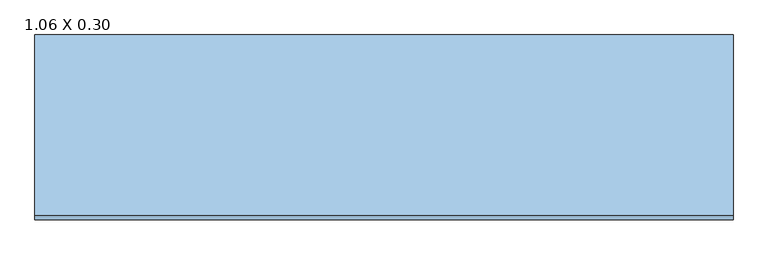
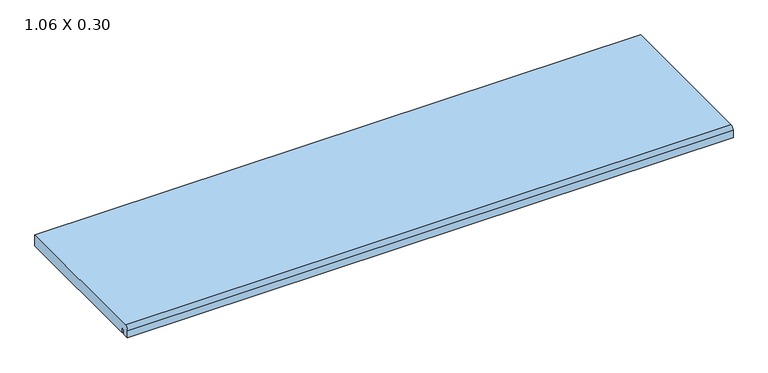
"""IFC4 building model written with IfcOpenShell, lengths in millimetres: window geometry, .CC_ND 300_PEDRA_PEITORIL RETO : 1.06 X 0.30."""

import ifcopenshell
import ifcopenshell.guid

model = None  # the IFC model being written
_history = None  # IfcOwnerHistory: only IFC2X3 demands one
_inside = {}  # id of a spatial element -> (the spatial element, [elements in it])
_under = {}  # id of a project, library or spatial element -> (it, [spatial elements below it])
_declared = {}  # id of a project -> (the project, [libraries it declares])
_typed = {}  # id of a type object -> (the type object, [elements of that type])
_made_of = {}  # id of a material, layer set ... -> (it, [elements and type objects made of it])


def new_model(schema):
    """Start an empty IFC model of exactly this schema.

    Asked for "IFC4X3", IfcOpenShell would pick the latest addendum, in which some entities
    have other attributes; the version numbers below select the first issue.
    IFC2X3 requires an IfcOwnerHistory on every rooted entity: one is made here for all.
    """
    global model, _history
    if schema == "IFC4X3":
        model = ifcopenshell.file(schema_version=(4, 3, 0, 0))
    else:
        model = ifcopenshell.file(schema=schema)
    _inside.clear()
    _under.clear()
    _declared.clear()
    _typed.clear()
    _made_of.clear()
    _history = None
    if model.schema == "IFC2X3":
        org = make("IfcOrganization", Name="unknown")
        user = make(
            "IfcPersonAndOrganization",
            ThePerson=make("IfcPerson", FamilyName="unknown"),
            TheOrganization=org,
        )
        app = make(
            "IfcApplication",
            ApplicationDeveloper=org,
            Version="unknown",
            ApplicationFullName="unknown",
            ApplicationIdentifier="unknown",
        )
        _history = make(
            "IfcOwnerHistory",
            OwningUser=user,
            OwningApplication=app,
            ChangeAction="ADDED",
            CreationDate=0,
        )
    return model


def make(cls, **values):
    """One entity of the class cls with the attributes given. An attribute that is None is left unset."""
    return model.create_entity(
        cls, **{name: value for name, value in values.items() if value is not None}
    )


def rooted(cls, **values):
    """An entity with a GlobalId (a new one), such as an element, a storey or a relation."""
    return make(cls, GlobalId=ifcopenshell.guid.new(), OwnerHistory=_history, **values)


def si_unit(unit_type, name, prefix=None):
    """IfcSIUnit, for example si_unit("LENGTHUNIT", "METRE", prefix="MILLI")."""
    return make("IfcSIUnit", UnitType=unit_type, Prefix=prefix, Name=name)


def assignment(units):
    """IfcUnitAssignment: the units of a project."""
    return None if units is None else make("IfcUnitAssignment", Units=units)


def point(xyz):
    """IfcCartesianPoint."""
    return None if xyz is None else make("IfcCartesianPoint", Coordinates=xyz)


def direction(xyz):
    """IfcDirection."""
    return None if xyz is None else make("IfcDirection", DirectionRatios=xyz)


def frame(location, z_axis=None, x_axis=None):
    """IfcAxis2Placement3D, a coordinate frame: its origin and axes. An axis left out is left unset."""
    return make(
        "IfcAxis2Placement3D",
        Location=point(location),
        Axis=direction(z_axis),
        RefDirection=direction(x_axis),
    )


def frame_2d(location, x_axis=None):
    """IfcAxis2Placement2D, a coordinate frame in the plane: its origin and x axis."""
    return make(
        "IfcAxis2Placement2D", Location=point(location), RefDirection=direction(x_axis)
    )


def origin():
    """The frame at (0, 0, 0) with its axes left unset."""
    return frame((0.0, 0.0, 0.0))


def place(relative_to, where):
    """IfcLocalPlacement: puts the frame where relative to a parent placement (None: the world)."""
    return make(
        "IfcLocalPlacement", PlacementRelTo=relative_to, RelativePlacement=where
    )


def context(
    kind, dimensions, precision=None, world=None, true_north=None, identifier=None
):
    """IfcGeometricRepresentationContext, for example the 3D "Model" context."""
    return make(
        "IfcGeometricRepresentationContext",
        ContextIdentifier=identifier,
        ContextType=kind,
        CoordinateSpaceDimension=dimensions,
        Precision=precision,
        WorldCoordinateSystem=world,
        TrueNorth=true_north,
    )


def project(units=None, contexts=None):
    """IfcProject with its units and contexts."""
    return rooted(
        "IfcProject",
        Name="project",
        RepresentationContexts=contexts,
        UnitsInContext=assignment(units),
    )


def spatial(cls, under=None, at=None, **own):
    """A site, building, storey or space (cls), placed at a placement, below another one or the project."""
    s = rooted(cls, ObjectPlacement=at, **own)
    if under is not None:
        _under.setdefault(under.id(), (under, []))[1].append(s)
    return s


def polyline(points):
    """IfcPolyline through the points."""
    return make("IfcPolyline", Points=[point(p) for p in points])


def circle_curve(where, radius):
    """IfcCircle in the frame where."""
    return make("IfcCircle", Position=where, Radius=radius)


def trimmed(basis, trim1, trim2, sense, master):
    """IfcTrimmedCurve: the piece of a basis curve between two trims."""
    return make(
        "IfcTrimmedCurve",
        BasisCurve=basis,
        Trim1=trim1,
        Trim2=trim2,
        SenseAgreement=sense,
        MasterRepresentation=master,
    )


def segment(curve, same_sense, transition):
    """IfcCompositeCurveSegment."""
    return make(
        "IfcCompositeCurveSegment",
        Transition=transition,
        SameSense=same_sense,
        ParentCurve=curve,
    )


def composite_curve(segments, self_intersect=None):
    """IfcCompositeCurve: segments joined end to end."""
    return make("IfcCompositeCurve", Segments=segments, SelfIntersect=self_intersect)


def outline(outer, holes=None, kind="AREA"):
    """IfcArbitraryClosedProfileDef: a profile drawn as a closed curve; with holes, ...WithVoids."""
    if holes is None:
        return make("IfcArbitraryClosedProfileDef", ProfileType=kind, OuterCurve=outer)
    return make(
        "IfcArbitraryProfileDefWithVoids",
        ProfileType=kind,
        OuterCurve=outer,
        InnerCurves=holes,
    )


def extrude(swept, where, along, depth):
    """IfcExtrudedAreaSolid: the profile swept, set in the frame where, extruded along a direction by depth."""
    return make(
        "IfcExtrudedAreaSolid",
        SweptArea=swept,
        Position=where,
        ExtrudedDirection=direction(along),
        Depth=depth,
    )


def shape(context_of_items, identifier, shape_type, items):
    """IfcShapeRepresentation: the items that make up one representation, for example the "Body"."""
    return make(
        "IfcShapeRepresentation",
        ContextOfItems=context_of_items,
        RepresentationIdentifier=identifier,
        RepresentationType=shape_type,
        Items=items,
    )


def source(mapping_origin, context_of_items, identifier, shape_type, items):
    """IfcRepresentationMap: a shape defined once, which mapped items show again and again."""
    return make(
        "IfcRepresentationMap",
        MappingOrigin=mapping_origin,
        MappedRepresentation=shape(context_of_items, identifier, shape_type, items),
    )


def transform(
    local_origin,
    x_axis=None,
    y_axis=None,
    z_axis=None,
    scale=None,
    scale2=None,
    scale3=None,
    uniform=True,
):
    """IfcCartesianTransformationOperator3D, or its non-uniform kind. x_axis, y_axis, z_axis: its Axis1, 2, 3."""
    if uniform:
        return make(
            "IfcCartesianTransformationOperator3D",
            Axis1=direction(x_axis),
            Axis2=direction(y_axis),
            LocalOrigin=point(local_origin),
            Scale=scale,
            Axis3=direction(z_axis),
        )
    return make(
        "IfcCartesianTransformationOperator3DnonUniform",
        Axis1=direction(x_axis),
        Axis2=direction(y_axis),
        LocalOrigin=point(local_origin),
        Scale=scale,
        Axis3=direction(z_axis),
        Scale2=scale2,
        Scale3=scale3,
    )


def mapped(mapping_source, mapping_target):
    """IfcMappedItem: shows the shape of a source again, moved by a transform."""
    return make(
        "IfcMappedItem", MappingSource=mapping_source, MappingTarget=mapping_target
    )


def made_of(thing, what):
    """Note that an element or type object is made of a material, layer set ...; save() writes the relation."""
    if what is not None:
        _made_of.setdefault(what.id(), (what, []))[1].append(thing)
    return thing


def element(
    cls,
    number,
    at=None,
    inside=None,
    cuts=None,
    type_object=None,
    material=None,
    context=None,
    identifier="Body",
    shape_type=None,
    held_by="IfcProductDefinitionShape",
    body=None,
    shapes=None,
    **own,
):
    """One element of the class cls, such as IfcWall. Its Tag is "e" and its number.

    at: its placement. inside: the storey or other place that contains it. cuts: it is an
    opening in that element (IfcRelVoidsElement). A single representation is given by context,
    identifier, shape_type and body (its items); several are given by shapes. held_by: the class
    of the entity that holds the representations. save() writes the other relations.
    """
    e = rooted(cls, Tag="e%d" % number, ObjectPlacement=at, **own)
    if body is not None:
        shapes = [shape(context, identifier, shape_type, body)]
    if shapes is not None:
        e.Representation = make(held_by, Representations=shapes)
    if inside is not None:
        _inside.setdefault(inside.id(), (inside, []))[1].append(e)
    if cuts is not None:
        rooted(
            "IfcRelVoidsElement", RelatingBuildingElement=cuts, RelatedOpeningElement=e
        )
    if type_object is not None:
        _typed.setdefault(type_object.id(), (type_object, []))[1].append(e)
    return made_of(e, material)


def aggregate(whole, parts):
    """IfcRelAggregates: a whole, such as a stair, and the parts it consists of."""
    return rooted("IfcRelAggregates", RelatingObject=whole, RelatedObjects=parts)


def save(model, path):
    """Write the relations noted so far, then the file.

    IfcRelAggregates (storeys below a building ...), IfcRelContainedInSpatialStructure (elements
    in a storey), IfcRelDefinesByType, IfcRelAssociatesMaterial and IfcRelDeclares: one each for
    every whole, place, type object, material and project.
    """
    for whole, parts in _under.values():
        aggregate(whole, parts)
    for where, things in _inside.values():
        rooted(
            "IfcRelContainedInSpatialStructure",
            RelatedElements=things,
            RelatingStructure=where,
        )
    for kind, things in _typed.values():
        rooted("IfcRelDefinesByType", RelatedObjects=things, RelatingType=kind)
    for what, things in _made_of.values():
        rooted("IfcRelAssociatesMaterial", RelatedObjects=things, RelatingMaterial=what)
    for by, libraries in _declared.values():
        rooted("IfcRelDeclares", RelatingContext=by, RelatedDefinitions=libraries)
    model.write(path)


def window_1_06_x_0_30_ddfe798f(model_context):
    return source(origin(), model_context, "Body", "SweptSolid", [
        extrude(outline(composite_curve([segment(polyline([(-132.5083081, 1480.0), (-132.5083081, 1488.1993124), (-137.2619526, 1488.1993124), (-137.2619526, 1480.0), (-148.0, 1480.0), (-148.0, 1493.3808343)]), True, "CONTINUOUS"), segment(trimmed(circle_curve(frame_2d((-141.3808343, 1493.3808343)), 6.6191657), [point((-148.0, 1493.3808343))], [point((-141.3808343, 1500.0))], False, "CARTESIAN"), True, "CONTINUOUS"), segment(polyline([(-141.3808343, 1500.0), (132.7, 1500.0), (132.7, 1480.0), (-132.5083081, 1480.0)]), True, "CONTINUOUS")], self_intersect=False)), frame((-530.0, 0.0, 0.0), z_axis=(1.0, 0.0, 0.0), x_axis=(0.0, 1.0, 0.0)), (0.0, 0.0, 1.0), 1060.0),
    ])


if __name__ == "__main__":
    model = new_model("IFC4")
    model_context = context("Model", 3, world=origin())
    ifc_project = project(units=[si_unit("LENGTHUNIT", "METRE", prefix="MILLI")], contexts=[model_context])
    site = spatial("IfcSite", under=ifc_project)
    building = spatial("IfcBuilding", under=site)
    placement = place(None, origin())
    window_1_06_x_0_30_shape = window_1_06_x_0_30_ddfe798f(model_context)
    element("IfcWindow", 1, ObjectType=".CC_ND 300_PEDRA_PEITORIL RETO : 1.06 X 0.30", at=placement, inside=building, context=model_context, shape_type="MappedRepresentation", body=[
        mapped(window_1_06_x_0_30_shape, transform((0.0, 0.0, 0.0), x_axis=(1.0, 0.0, 0.0), y_axis=(0.0, 1.0, 0.0), z_axis=(0.0, 0.0, 1.0))),
    ])
    save(model, "model.ifc")

# Revit data of these elements
# Type ".CC_ND 300_PEDRA_PEITORIL RETO : 1.06 X 0.30"
#   Type Mark = "68"
#   Largura da pedra [instance default] = 0.26 m
#   Extensão interior peitoril [instance default] = 0.03 m
#   Extensão exterior peitoril [instance default] = 0.03 m
#   Espessura = 0.02 m
#   Comprimento = 1.06 m
#   Altura-padrão do peitoril = 1.48 m
#   Peitoril = .GRANITO_BRANCO_ITAUNAS
#   Rough Width = 0
#   Rough Height = 0
#   Height = 0
#   Wall Closure = (empty or 0)
#   Width = 0
# Element 1 (IfcWindow, ".CC_ND 300_PEDRA_PEITORIL RETO : 1.06 X 0.30")
#   Largura da pedra = 0.2807 m
#   Extensão interior peitoril = 0.0147 m
#   Materials on its faces: ".GRANITO_BRANCO_ITAUNAS"
# Materials
#   ".GRANITO_BRANCO_ITAUNAS": class ".CC_PEDRA REVEST.", colour RGB 202 195 174, transparency 0, Description = "Revestimento em granito", Cost = 0
